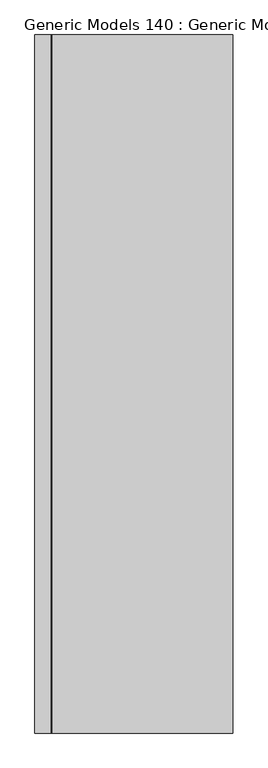
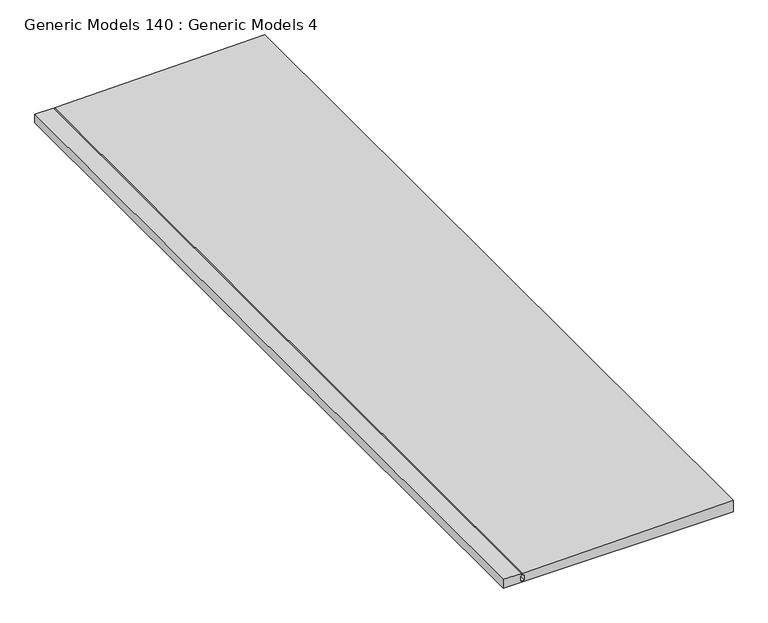
"""IFC4 building model written with IfcOpenShell, lengths in millimetres: proxy geometry, Generic Models 140 : Generic Models 4."""

import ifcopenshell
import ifcopenshell.guid

model = None  # the IFC model being written
_history = None  # IfcOwnerHistory: only IFC2X3 demands one
_inside = {}  # id of a spatial element -> (the spatial element, [elements in it])
_under = {}  # id of a project, library or spatial element -> (it, [spatial elements below it])
_declared = {}  # id of a project -> (the project, [libraries it declares])
_typed = {}  # id of a type object -> (the type object, [elements of that type])
_made_of = {}  # id of a material, layer set ... -> (it, [elements and type objects made of it])


def new_model(schema):
    """Start an empty IFC model of exactly this schema.

    Asked for "IFC4X3", IfcOpenShell would pick the latest addendum, in which some entities
    have other attributes; the version numbers below select the first issue.
    IFC2X3 requires an IfcOwnerHistory on every rooted entity: one is made here for all.
    """
    global model, _history
    if schema == "IFC4X3":
        model = ifcopenshell.file(schema_version=(4, 3, 0, 0))
    else:
        model = ifcopenshell.file(schema=schema)
    _inside.clear()
    _under.clear()
    _declared.clear()
    _typed.clear()
    _made_of.clear()
    _history = None
    if model.schema == "IFC2X3":
        org = make("IfcOrganization", Name="unknown")
        user = make(
            "IfcPersonAndOrganization",
            ThePerson=make("IfcPerson", FamilyName="unknown"),
            TheOrganization=org,
        )
        app = make(
            "IfcApplication",
            ApplicationDeveloper=org,
            Version="unknown",
            ApplicationFullName="unknown",
            ApplicationIdentifier="unknown",
        )
        _history = make(
            "IfcOwnerHistory",
            OwningUser=user,
            OwningApplication=app,
            ChangeAction="ADDED",
            CreationDate=0,
        )
    return model


def make(cls, **values):
    """One entity of the class cls with the attributes given. An attribute that is None is left unset."""
    return model.create_entity(
        cls, **{name: value for name, value in values.items() if value is not None}
    )


def rooted(cls, **values):
    """An entity with a GlobalId (a new one), such as an element, a storey or a relation."""
    return make(cls, GlobalId=ifcopenshell.guid.new(), OwnerHistory=_history, **values)


def si_unit(unit_type, name, prefix=None):
    """IfcSIUnit, for example si_unit("LENGTHUNIT", "METRE", prefix="MILLI")."""
    return make("IfcSIUnit", UnitType=unit_type, Prefix=prefix, Name=name)


def assignment(units):
    """IfcUnitAssignment: the units of a project."""
    return None if units is None else make("IfcUnitAssignment", Units=units)


def point(xyz):
    """IfcCartesianPoint."""
    return None if xyz is None else make("IfcCartesianPoint", Coordinates=xyz)


def direction(xyz):
    """IfcDirection."""
    return None if xyz is None else make("IfcDirection", DirectionRatios=xyz)


def frame(location, z_axis=None, x_axis=None):
    """IfcAxis2Placement3D, a coordinate frame: its origin and axes. An axis left out is left unset."""
    return make(
        "IfcAxis2Placement3D",
        Location=point(location),
        Axis=direction(z_axis),
        RefDirection=direction(x_axis),
    )


def origin():
    """The frame at (0, 0, 0) with its axes left unset."""
    return frame((0.0, 0.0, 0.0))


def place(relative_to, where):
    """IfcLocalPlacement: puts the frame where relative to a parent placement (None: the world)."""
    return make(
        "IfcLocalPlacement", PlacementRelTo=relative_to, RelativePlacement=where
    )


def context(
    kind, dimensions, precision=None, world=None, true_north=None, identifier=None
):
    """IfcGeometricRepresentationContext, for example the 3D "Model" context."""
    return make(
        "IfcGeometricRepresentationContext",
        ContextIdentifier=identifier,
        ContextType=kind,
        CoordinateSpaceDimension=dimensions,
        Precision=precision,
        WorldCoordinateSystem=world,
        TrueNorth=true_north,
    )


def project(units=None, contexts=None):
    """IfcProject with its units and contexts."""
    return rooted(
        "IfcProject",
        Name="project",
        RepresentationContexts=contexts,
        UnitsInContext=assignment(units),
    )


def spatial(cls, under=None, at=None, **own):
    """A site, building, storey or space (cls), placed at a placement, below another one or the project."""
    s = rooted(cls, ObjectPlacement=at, **own)
    if under is not None:
        _under.setdefault(under.id(), (under, []))[1].append(s)
    return s


def polyline(points):
    """IfcPolyline through the points."""
    return make("IfcPolyline", Points=[point(p) for p in points])


def outline(outer, holes=None, kind="AREA"):
    """IfcArbitraryClosedProfileDef: a profile drawn as a closed curve; with holes, ...WithVoids."""
    if holes is None:
        return make("IfcArbitraryClosedProfileDef", ProfileType=kind, OuterCurve=outer)
    return make(
        "IfcArbitraryProfileDefWithVoids",
        ProfileType=kind,
        OuterCurve=outer,
        InnerCurves=holes,
    )


def extrude(swept, where, along, depth):
    """IfcExtrudedAreaSolid: the profile swept, set in the frame where, extruded along a direction by depth."""
    return make(
        "IfcExtrudedAreaSolid",
        SweptArea=swept,
        Position=where,
        ExtrudedDirection=direction(along),
        Depth=depth,
    )


def shape(context_of_items, identifier, shape_type, items):
    """IfcShapeRepresentation: the items that make up one representation, for example the "Body"."""
    return make(
        "IfcShapeRepresentation",
        ContextOfItems=context_of_items,
        RepresentationIdentifier=identifier,
        RepresentationType=shape_type,
        Items=items,
    )


def source(mapping_origin, context_of_items, identifier, shape_type, items):
    """IfcRepresentationMap: a shape defined once, which mapped items show again and again."""
    return make(
        "IfcRepresentationMap",
        MappingOrigin=mapping_origin,
        MappedRepresentation=shape(context_of_items, identifier, shape_type, items),
    )


def transform(
    local_origin,
    x_axis=None,
    y_axis=None,
    z_axis=None,
    scale=None,
    scale2=None,
    scale3=None,
    uniform=True,
):
    """IfcCartesianTransformationOperator3D, or its non-uniform kind. x_axis, y_axis, z_axis: its Axis1, 2, 3."""
    if uniform:
        return make(
            "IfcCartesianTransformationOperator3D",
            Axis1=direction(x_axis),
            Axis2=direction(y_axis),
            LocalOrigin=point(local_origin),
            Scale=scale,
            Axis3=direction(z_axis),
        )
    return make(
        "IfcCartesianTransformationOperator3DnonUniform",
        Axis1=direction(x_axis),
        Axis2=direction(y_axis),
        LocalOrigin=point(local_origin),
        Scale=scale,
        Axis3=direction(z_axis),
        Scale2=scale2,
        Scale3=scale3,
    )


def mapped(mapping_source, mapping_target):
    """IfcMappedItem: shows the shape of a source again, moved by a transform."""
    return make(
        "IfcMappedItem", MappingSource=mapping_source, MappingTarget=mapping_target
    )


def made_of(thing, what):
    """Note that an element or type object is made of a material, layer set ...; save() writes the relation."""
    if what is not None:
        _made_of.setdefault(what.id(), (what, []))[1].append(thing)
    return thing


def element(
    cls,
    number,
    at=None,
    inside=None,
    cuts=None,
    type_object=None,
    material=None,
    context=None,
    identifier="Body",
    shape_type=None,
    held_by="IfcProductDefinitionShape",
    body=None,
    shapes=None,
    **own,
):
    """One element of the class cls, such as IfcWall. Its Tag is "e" and its number.

    at: its placement. inside: the storey or other place that contains it. cuts: it is an
    opening in that element (IfcRelVoidsElement). A single representation is given by context,
    identifier, shape_type and body (its items); several are given by shapes. held_by: the class
    of the entity that holds the representations. save() writes the other relations.
    """
    e = rooted(cls, Tag="e%d" % number, ObjectPlacement=at, **own)
    if body is not None:
        shapes = [shape(context, identifier, shape_type, body)]
    if shapes is not None:
        e.Representation = make(held_by, Representations=shapes)
    if inside is not None:
        _inside.setdefault(inside.id(), (inside, []))[1].append(e)
    if cuts is not None:
        rooted(
            "IfcRelVoidsElement", RelatingBuildingElement=cuts, RelatedOpeningElement=e
        )
    if type_object is not None:
        _typed.setdefault(type_object.id(), (type_object, []))[1].append(e)
    return made_of(e, material)


def aggregate(whole, parts):
    """IfcRelAggregates: a whole, such as a stair, and the parts it consists of."""
    return rooted("IfcRelAggregates", RelatingObject=whole, RelatedObjects=parts)


def save(model, path):
    """Write the relations noted so far, then the file.

    IfcRelAggregates (storeys below a building ...), IfcRelContainedInSpatialStructure (elements
    in a storey), IfcRelDefinesByType, IfcRelAssociatesMaterial and IfcRelDeclares: one each for
    every whole, place, type object, material and project.
    """
    for whole, parts in _under.values():
        aggregate(whole, parts)
    for where, things in _inside.values():
        rooted(
            "IfcRelContainedInSpatialStructure",
            RelatedElements=things,
            RelatingStructure=where,
        )
    for kind, things in _typed.values():
        rooted("IfcRelDefinesByType", RelatedObjects=things, RelatingType=kind)
    for what, things in _made_of.values():
        rooted("IfcRelAssociatesMaterial", RelatedObjects=things, RelatingMaterial=what)
    for by, libraries in _declared.values():
        rooted("IfcRelDeclares", RelatingContext=by, RelatedDefinitions=libraries)
    model.write(path)


def generic_models_140_generic_models_4_92953a17(model_context):
    return source(origin(), model_context, "Body", "SweptSolid", [
        extrude(outline(polyline([(122955.6484874, -10290.0847239), (122955.6484874, -6731.1736296), (123149.8368207, -6731.1736296), (123093.0827884, -9982.6099618), (123062.8101831, -9982.6099618), (123052.998594, -9964.236761), (122977.7455153, -9964.236761), (122964.4770394, -9994.8097239), (122979.3364482, -10024.561761), (123054.6250157, -10024.561761), (123062.917352, -10005.4547218), (123093.0827884, -10005.4547218), (123098.0510236, -10290.0847239), (122955.6484874, -10290.0847239)])), frame((0.0, -5493.3230338, 0.0), z_axis=(0.0, 1.0, 0.0), x_axis=(0.0, 0.0, 1.0)), (0.0, 0.0, 1.0), 12547.6),
    ])


if __name__ == "__main__":
    model = new_model("IFC4")
    model_context = context("Model", 3, world=origin())
    ifc_project = project(units=[si_unit("LENGTHUNIT", "METRE", prefix="MILLI")], contexts=[model_context])
    site = spatial("IfcSite", under=ifc_project)
    building = spatial("IfcBuilding", under=site)
    placement = place(None, origin())
    generic_models_140_generic_models_4_shape = generic_models_140_generic_models_4_92953a17(model_context)
    element("IfcBuildingElementProxy", 1, Name="Generic Models 140 : Generic Models 4", ObjectType="Generic Models 140 : Generic Models 4", at=placement, inside=building, context=model_context, shape_type="MappedRepresentation", body=[
        mapped(generic_models_140_generic_models_4_shape, transform((0.0, 0.0, 0.0), x_axis=(1.0, 0.0, 0.0), y_axis=(0.0, 1.0, 0.0), z_axis=(0.0, 0.0, 1.0))),
    ])
    save(model, "model.ifc")

# Revit data of these elements
# Element 1 (IfcBuildingElementProxy, "Generic Models 140 : Generic Models 4")
#   Materials on its faces: "_CONCRETE SLAB W/ WIRE MESH (SEE STRUCT. DWGS) - SLOPE 1% AWAY FROM BUILDING"
# Materials
#   "_CONCRETE SLAB W/ WIRE MESH (SEE STRUCT. DWGS) - SLOPE 1% AWAY FROM BUILDING": class "Generic", colour RGB 191 191 191, transparency 0, Cost = 0
